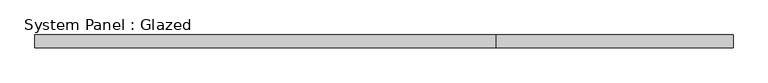
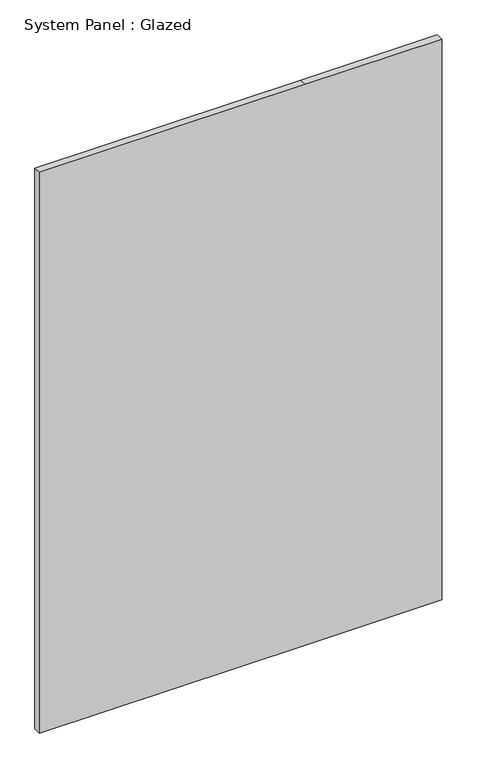
"""IFC4 building model written with IfcOpenShell, lengths in millimetres: plate geometry, System Panel : Glazed."""

from ifc_helpers import new_model, si_unit, frame, origin, place, context, project, spatial, polyline, outline, extrude, source, transform, mapped, element, save


def system_panel_glazed_b9816be8(model_context):
    return source(origin(), model_context, "Body", "SweptSolid", [
        extrude(outline(polyline([(0.0, -692.15), (0.0, 222.25), (0.0, 692.15), (2038.35, 692.15), (2038.35, 222.25), (2038.35, -692.15), (0.0, -692.15)])), frame((0.0, -44.45, 0.0), z_axis=(0.0, 1.0, 0.0), x_axis=(0.0, 0.0, 1.0)), (0.0, 0.0, 1.0), 25.4),
    ])


if __name__ == "__main__":
    model = new_model("IFC4")
    model_context = context("Model", 3, world=origin())
    ifc_project = project(units=[si_unit("LENGTHUNIT", "METRE", prefix="MILLI")], contexts=[model_context])
    site = spatial("IfcSite", under=ifc_project)
    building = spatial("IfcBuilding", under=site)
    placement = place(None, origin())
    system_panel_glazed_shape = system_panel_glazed_b9816be8(model_context)
    element("IfcPlate", 1, ObjectType="System Panel : Glazed", at=placement, inside=building, context=model_context, shape_type="MappedRepresentation", body=[
        mapped(system_panel_glazed_shape, transform((0.0, 0.0, 0.0), x_axis=(1.0, 0.0, 0.0), y_axis=(0.0, 1.0, 0.0), z_axis=(0.0, 0.0, 1.0))),
    ])
    save(model, "model.ifc")

# Revit data of these elements
# Type "System Panel : Glazed"
#   Construction Type Id = "GSP4R"
#   Analytic Construction = "1/8 in Pilkington single glazing"
#   Visual Light Transmittance = 0.9
#   Solar Heat Gain Coefficient = 0.86
#   Heat Transfer Coefficient (U) = 1.18115 BTU/(h·ft²·°F)
#   Define Thermal Properties by = 1
# Element 1 (IfcPlate, "System Panel : Glazed")
#   Materials on its faces: "Glass"
# Materials
#   "Glass": class "Glass", colour RGB 0 0 255, transparency 0.75, Description = "Soda Lime Glass", Cost = 0
